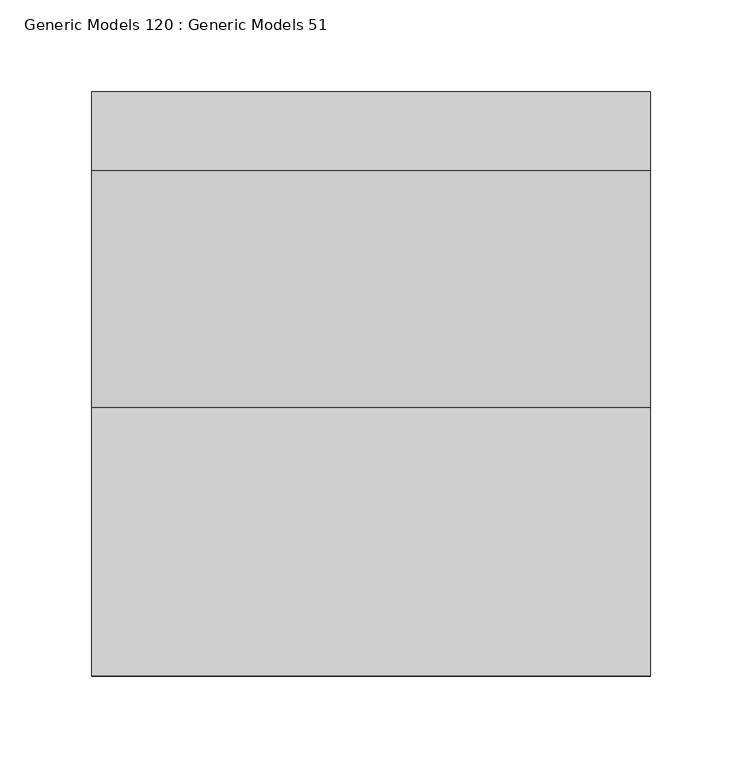
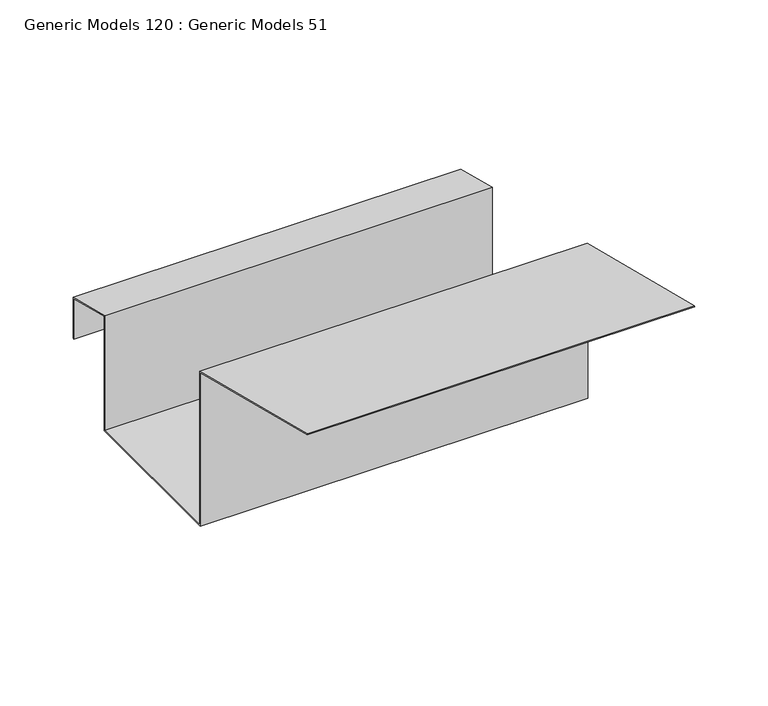
"""IFC4 building model written with IfcOpenShell, lengths in millimetres: proxy geometry, Generic Models 120 : Generic Models 51."""

from ifc_helpers import new_model, si_unit, frame, origin, place, context, project, spatial, polyline, outline, extrude, source, transform, mapped, element, save


def generic_models_120_generic_models_51_4fbcd6bf(model_context):
    return source(origin(), model_context, "Body", "SweptSolid", [
        extrude(outline(polyline([(12460.130277, 129618.2048417), (12314.5772632, 129654.5930952), (12314.7697758, 129655.3631458), (12460.924027, 129618.824583), (12460.924027, 129490.9736742), (12590.6832162, 129490.9736742), (12590.6832162, 129586.4458779), (12633.3849613, 129575.7991371), (12633.3849613, 129541.5233269), (12632.5912113, 129541.5233269), (12632.5912113, 129575.1789916), (12591.4769662, 129585.4299242), (12591.4769662, 129490.1799242), (12460.130277, 129490.1799242), (12460.130277, 129618.2048417)])), frame((1084.7910488, 0.0, 0.0), z_axis=(1.0, 0.0, 0.0), x_axis=(0.0, 1.0, 0.0)), (0.0, 0.0, 1.0), 304.8),
    ])


if __name__ == "__main__":
    model = new_model("IFC4")
    model_context = context("Model", 3, world=origin())
    ifc_project = project(units=[si_unit("LENGTHUNIT", "METRE", prefix="MILLI")], contexts=[model_context])
    site = spatial("IfcSite", under=ifc_project)
    building = spatial("IfcBuilding", under=site)
    placement = place(None, origin())
    generic_models_120_generic_models_51_shape = generic_models_120_generic_models_51_4fbcd6bf(model_context)
    element("IfcBuildingElementProxy", 1, Name="Generic Models 120 : Generic Models 51", ObjectType="Generic Models 120 : Generic Models 51", at=placement, inside=building, context=model_context, shape_type="MappedRepresentation", body=[
        mapped(generic_models_120_generic_models_51_shape, transform((0.0, 0.0, 0.0), x_axis=(1.0, 0.0, 0.0), y_axis=(0.0, 1.0, 0.0), z_axis=(0.0, 0.0, 1.0))),
    ])
    save(model, "model.ifc")

# Revit data of these elements
# Element 1 (IfcBuildingElementProxy, "Generic Models 120 : Generic Models 51")
#   Materials on its faces: "_SELF ADHERED MEMBRANE W/ END DAMS WHERE POSSIBLE"
# Materials
#   "_SELF ADHERED MEMBRANE W/ END DAMS WHERE POSSIBLE": class "Generic", colour RGB 253 192 103, transparency 0, Cost = 0
